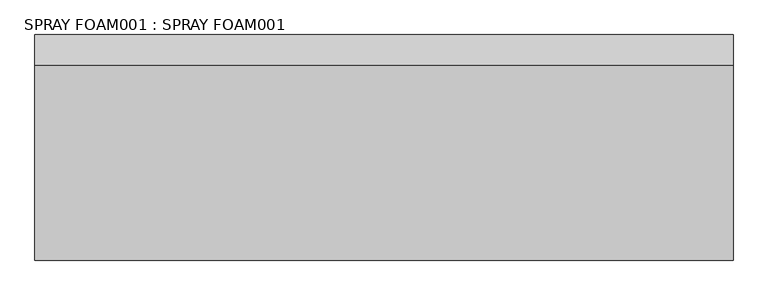
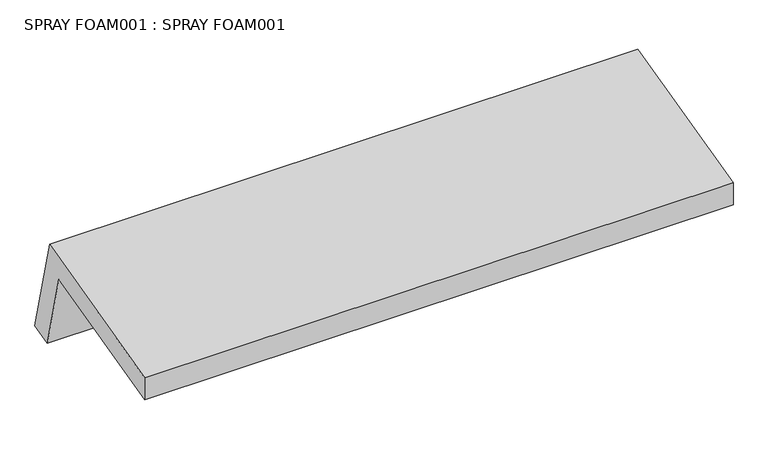
"""IFC4 building model written with IfcOpenShell, lengths in millimetres: proxy geometry, SPRAY FOAM001 : SPRAY FOAM001."""

import ifcopenshell
import ifcopenshell.guid

model = None  # the IFC model being written
_history = None  # IfcOwnerHistory: only IFC2X3 demands one
_inside = {}  # id of a spatial element -> (the spatial element, [elements in it])
_under = {}  # id of a project, library or spatial element -> (it, [spatial elements below it])
_declared = {}  # id of a project -> (the project, [libraries it declares])
_typed = {}  # id of a type object -> (the type object, [elements of that type])
_made_of = {}  # id of a material, layer set ... -> (it, [elements and type objects made of it])


def new_model(schema):
    """Start an empty IFC model of exactly this schema.

    Asked for "IFC4X3", IfcOpenShell would pick the latest addendum, in which some entities
    have other attributes; the version numbers below select the first issue.
    IFC2X3 requires an IfcOwnerHistory on every rooted entity: one is made here for all.
    """
    global model, _history
    if schema == "IFC4X3":
        model = ifcopenshell.file(schema_version=(4, 3, 0, 0))
    else:
        model = ifcopenshell.file(schema=schema)
    _inside.clear()
    _under.clear()
    _declared.clear()
    _typed.clear()
    _made_of.clear()
    _history = None
    if model.schema == "IFC2X3":
        org = make("IfcOrganization", Name="unknown")
        user = make(
            "IfcPersonAndOrganization",
            ThePerson=make("IfcPerson", FamilyName="unknown"),
            TheOrganization=org,
        )
        app = make(
            "IfcApplication",
            ApplicationDeveloper=org,
            Version="unknown",
            ApplicationFullName="unknown",
            ApplicationIdentifier="unknown",
        )
        _history = make(
            "IfcOwnerHistory",
            OwningUser=user,
            OwningApplication=app,
            ChangeAction="ADDED",
            CreationDate=0,
        )
    return model


def make(cls, **values):
    """One entity of the class cls with the attributes given. An attribute that is None is left unset."""
    return model.create_entity(
        cls, **{name: value for name, value in values.items() if value is not None}
    )


def rooted(cls, **values):
    """An entity with a GlobalId (a new one), such as an element, a storey or a relation."""
    return make(cls, GlobalId=ifcopenshell.guid.new(), OwnerHistory=_history, **values)


def si_unit(unit_type, name, prefix=None):
    """IfcSIUnit, for example si_unit("LENGTHUNIT", "METRE", prefix="MILLI")."""
    return make("IfcSIUnit", UnitType=unit_type, Prefix=prefix, Name=name)


def assignment(units):
    """IfcUnitAssignment: the units of a project."""
    return None if units is None else make("IfcUnitAssignment", Units=units)


def point(xyz):
    """IfcCartesianPoint."""
    return None if xyz is None else make("IfcCartesianPoint", Coordinates=xyz)


def direction(xyz):
    """IfcDirection."""
    return None if xyz is None else make("IfcDirection", DirectionRatios=xyz)


def frame(location, z_axis=None, x_axis=None):
    """IfcAxis2Placement3D, a coordinate frame: its origin and axes. An axis left out is left unset."""
    return make(
        "IfcAxis2Placement3D",
        Location=point(location),
        Axis=direction(z_axis),
        RefDirection=direction(x_axis),
    )


def origin():
    """The frame at (0, 0, 0) with its axes left unset."""
    return frame((0.0, 0.0, 0.0))


def place(relative_to, where):
    """IfcLocalPlacement: puts the frame where relative to a parent placement (None: the world)."""
    return make(
        "IfcLocalPlacement", PlacementRelTo=relative_to, RelativePlacement=where
    )


def context(
    kind, dimensions, precision=None, world=None, true_north=None, identifier=None
):
    """IfcGeometricRepresentationContext, for example the 3D "Model" context."""
    return make(
        "IfcGeometricRepresentationContext",
        ContextIdentifier=identifier,
        ContextType=kind,
        CoordinateSpaceDimension=dimensions,
        Precision=precision,
        WorldCoordinateSystem=world,
        TrueNorth=true_north,
    )


def project(units=None, contexts=None):
    """IfcProject with its units and contexts."""
    return rooted(
        "IfcProject",
        Name="project",
        RepresentationContexts=contexts,
        UnitsInContext=assignment(units),
    )


def spatial(cls, under=None, at=None, **own):
    """A site, building, storey or space (cls), placed at a placement, below another one or the project."""
    s = rooted(cls, ObjectPlacement=at, **own)
    if under is not None:
        _under.setdefault(under.id(), (under, []))[1].append(s)
    return s


def polyline(points):
    """IfcPolyline through the points."""
    return make("IfcPolyline", Points=[point(p) for p in points])


def outline(outer, holes=None, kind="AREA"):
    """IfcArbitraryClosedProfileDef: a profile drawn as a closed curve; with holes, ...WithVoids."""
    if holes is None:
        return make("IfcArbitraryClosedProfileDef", ProfileType=kind, OuterCurve=outer)
    return make(
        "IfcArbitraryProfileDefWithVoids",
        ProfileType=kind,
        OuterCurve=outer,
        InnerCurves=holes,
    )


def extrude(swept, where, along, depth):
    """IfcExtrudedAreaSolid: the profile swept, set in the frame where, extruded along a direction by depth."""
    return make(
        "IfcExtrudedAreaSolid",
        SweptArea=swept,
        Position=where,
        ExtrudedDirection=direction(along),
        Depth=depth,
    )


def shape(context_of_items, identifier, shape_type, items):
    """IfcShapeRepresentation: the items that make up one representation, for example the "Body"."""
    return make(
        "IfcShapeRepresentation",
        ContextOfItems=context_of_items,
        RepresentationIdentifier=identifier,
        RepresentationType=shape_type,
        Items=items,
    )


def source(mapping_origin, context_of_items, identifier, shape_type, items):
    """IfcRepresentationMap: a shape defined once, which mapped items show again and again."""
    return make(
        "IfcRepresentationMap",
        MappingOrigin=mapping_origin,
        MappedRepresentation=shape(context_of_items, identifier, shape_type, items),
    )


def transform(
    local_origin,
    x_axis=None,
    y_axis=None,
    z_axis=None,
    scale=None,
    scale2=None,
    scale3=None,
    uniform=True,
):
    """IfcCartesianTransformationOperator3D, or its non-uniform kind. x_axis, y_axis, z_axis: its Axis1, 2, 3."""
    if uniform:
        return make(
            "IfcCartesianTransformationOperator3D",
            Axis1=direction(x_axis),
            Axis2=direction(y_axis),
            LocalOrigin=point(local_origin),
            Scale=scale,
            Axis3=direction(z_axis),
        )
    return make(
        "IfcCartesianTransformationOperator3DnonUniform",
        Axis1=direction(x_axis),
        Axis2=direction(y_axis),
        LocalOrigin=point(local_origin),
        Scale=scale,
        Axis3=direction(z_axis),
        Scale2=scale2,
        Scale3=scale3,
    )


def mapped(mapping_source, mapping_target):
    """IfcMappedItem: shows the shape of a source again, moved by a transform."""
    return make(
        "IfcMappedItem", MappingSource=mapping_source, MappingTarget=mapping_target
    )


def made_of(thing, what):
    """Note that an element or type object is made of a material, layer set ...; save() writes the relation."""
    if what is not None:
        _made_of.setdefault(what.id(), (what, []))[1].append(thing)
    return thing


def element(
    cls,
    number,
    at=None,
    inside=None,
    cuts=None,
    type_object=None,
    material=None,
    context=None,
    identifier="Body",
    shape_type=None,
    held_by="IfcProductDefinitionShape",
    body=None,
    shapes=None,
    **own,
):
    """One element of the class cls, such as IfcWall. Its Tag is "e" and its number.

    at: its placement. inside: the storey or other place that contains it. cuts: it is an
    opening in that element (IfcRelVoidsElement). A single representation is given by context,
    identifier, shape_type and body (its items); several are given by shapes. held_by: the class
    of the entity that holds the representations. save() writes the other relations.
    """
    e = rooted(cls, Tag="e%d" % number, ObjectPlacement=at, **own)
    if body is not None:
        shapes = [shape(context, identifier, shape_type, body)]
    if shapes is not None:
        e.Representation = make(held_by, Representations=shapes)
    if inside is not None:
        _inside.setdefault(inside.id(), (inside, []))[1].append(e)
    if cuts is not None:
        rooted(
            "IfcRelVoidsElement", RelatingBuildingElement=cuts, RelatedOpeningElement=e
        )
    if type_object is not None:
        _typed.setdefault(type_object.id(), (type_object, []))[1].append(e)
    return made_of(e, material)


def aggregate(whole, parts):
    """IfcRelAggregates: a whole, such as a stair, and the parts it consists of."""
    return rooted("IfcRelAggregates", RelatingObject=whole, RelatedObjects=parts)


def save(model, path):
    """Write the relations noted so far, then the file.

    IfcRelAggregates (storeys below a building ...), IfcRelContainedInSpatialStructure (elements
    in a storey), IfcRelDefinesByType, IfcRelAssociatesMaterial and IfcRelDeclares: one each for
    every whole, place, type object, material and project.
    """
    for whole, parts in _under.values():
        aggregate(whole, parts)
    for where, things in _inside.values():
        rooted(
            "IfcRelContainedInSpatialStructure",
            RelatedElements=things,
            RelatingStructure=where,
        )
    for kind, things in _typed.values():
        rooted("IfcRelDefinesByType", RelatedObjects=things, RelatingType=kind)
    for what, things in _made_of.values():
        rooted("IfcRelAssociatesMaterial", RelatedObjects=things, RelatingMaterial=what)
    for by, libraries in _declared.values():
        rooted("IfcRelDeclares", RelatingContext=by, RelatedDefinitions=libraries)
    model.write(path)


def spray_foam001_spray_foam001_9babf991(model_context):
    return source(origin(), model_context, "Body", "SweptSolid", [
        extrude(outline(polyline([(8857.5938813, 43384.4932401), (9417.6229917, 43524.5643553), (9503.8912781, 43179.5873376), (9429.9539501, 43161.1560729), (9362.1861979, 43432.1515684), (8857.5938813, 43305.9459708), (8857.5938813, 43384.4932401)])), frame((3700.3883192, 0.0, 0.0), z_axis=(1.0, 0.0, 0.0), x_axis=(0.0, 1.0, 0.0)), (0.0, 0.0, 1.0), 2000.25),
    ])


if __name__ == "__main__":
    model = new_model("IFC4")
    model_context = context("Model", 3, world=origin())
    ifc_project = project(units=[si_unit("LENGTHUNIT", "METRE", prefix="MILLI")], contexts=[model_context])
    site = spatial("IfcSite", under=ifc_project)
    building = spatial("IfcBuilding", under=site)
    placement = place(None, origin())
    spray_foam001_spray_foam001_shape = spray_foam001_spray_foam001_9babf991(model_context)
    element("IfcBuildingElementProxy", 1, Name="SPRAY FOAM001 : SPRAY FOAM001", ObjectType="SPRAY FOAM001 : SPRAY FOAM001", at=placement, inside=building, context=model_context, shape_type="MappedRepresentation", body=[
        mapped(spray_foam001_spray_foam001_shape, transform((0.0, 0.0, 0.0), x_axis=(1.0, 0.0, 0.0), y_axis=(0.0, 1.0, 0.0), z_axis=(0.0, 0.0, 1.0))),
    ])
    save(model, "model.ifc")

# Revit data of these elements
# Type "SPRAY FOAM001 : SPRAY FOAM001"
#   NameOverride = "SPRAY FOAM001"
# Element 1 (IfcBuildingElementProxy, "SPRAY FOAM001 : SPRAY FOAM001")
#   Materials on its faces: "3\" POLYURETHANE SPRAY FOAM UNDER ROOF SUBSTRATE"
# Materials
#   "3\" POLYURETHANE SPRAY FOAM UNDER ROOF SUBSTRATE": class "Unassigned", colour RGB 193 227 245, transparency 0
